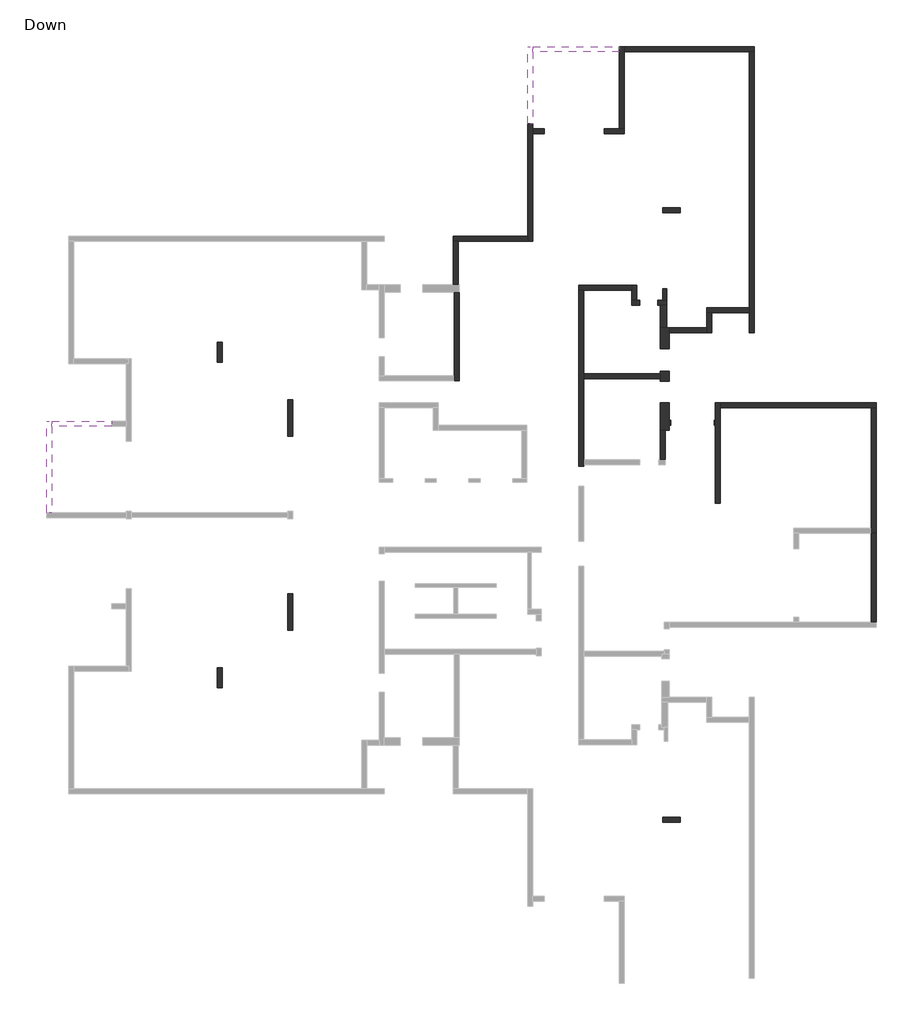
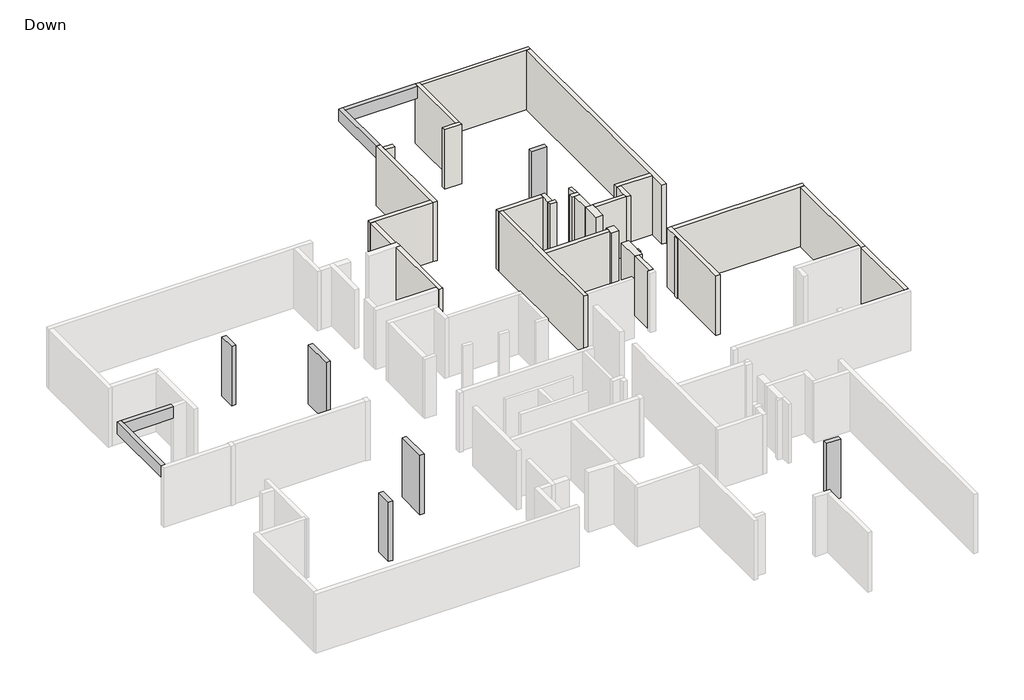
# One storey, part 3 of 3: 30 walls, 6 columns, 4 beams.
"""IFC4 building model written with IfcOpenShell, lengths in millimetres."""

import ifcopenshell
import ifcopenshell.guid

model = None  # the IFC model being written
_history = None  # IfcOwnerHistory: only IFC2X3 demands one
_inside = {}  # id of a spatial element -> (the spatial element, [elements in it])
_under = {}  # id of a project, library or spatial element -> (it, [spatial elements below it])
_declared = {}  # id of a project -> (the project, [libraries it declares])
_typed = {}  # id of a type object -> (the type object, [elements of that type])
_made_of = {}  # id of a material, layer set ... -> (it, [elements and type objects made of it])


def new_model(schema):
    """Start an empty IFC model of exactly this schema.

    Asked for "IFC4X3", IfcOpenShell would pick the latest addendum, in which some entities
    have other attributes; the version numbers below select the first issue.
    IFC2X3 requires an IfcOwnerHistory on every rooted entity: one is made here for all.
    """
    global model, _history
    if schema == "IFC4X3":
        model = ifcopenshell.file(schema_version=(4, 3, 0, 0))
    else:
        model = ifcopenshell.file(schema=schema)
    _inside.clear()
    _under.clear()
    _declared.clear()
    _typed.clear()
    _made_of.clear()
    _history = None
    if model.schema == "IFC2X3":
        org = make("IfcOrganization", Name="unknown")
        user = make(
            "IfcPersonAndOrganization",
            ThePerson=make("IfcPerson", FamilyName="unknown"),
            TheOrganization=org,
        )
        app = make(
            "IfcApplication",
            ApplicationDeveloper=org,
            Version="unknown",
            ApplicationFullName="unknown",
            ApplicationIdentifier="unknown",
        )
        _history = make(
            "IfcOwnerHistory",
            OwningUser=user,
            OwningApplication=app,
            ChangeAction="ADDED",
            CreationDate=0,
        )
    return model


def make(cls, **values):
    """One entity of the class cls with the attributes given. An attribute that is None is left unset."""
    return model.create_entity(
        cls, **{name: value for name, value in values.items() if value is not None}
    )


def rooted(cls, **values):
    """An entity with a GlobalId (a new one), such as an element, a storey or a relation."""
    return make(cls, GlobalId=ifcopenshell.guid.new(), OwnerHistory=_history, **values)


def si_unit(unit_type, name, prefix=None):
    """IfcSIUnit, for example si_unit("LENGTHUNIT", "METRE", prefix="MILLI")."""
    return make("IfcSIUnit", UnitType=unit_type, Prefix=prefix, Name=name)


def assignment(units):
    """IfcUnitAssignment: the units of a project."""
    return None if units is None else make("IfcUnitAssignment", Units=units)


def point(xyz):
    """IfcCartesianPoint."""
    return None if xyz is None else make("IfcCartesianPoint", Coordinates=xyz)


def direction(xyz):
    """IfcDirection."""
    return None if xyz is None else make("IfcDirection", DirectionRatios=xyz)


def frame(location, z_axis=None, x_axis=None):
    """IfcAxis2Placement3D, a coordinate frame: its origin and axes. An axis left out is left unset."""
    return make(
        "IfcAxis2Placement3D",
        Location=point(location),
        Axis=direction(z_axis),
        RefDirection=direction(x_axis),
    )


def origin():
    """The frame at (0, 0, 0) with its axes left unset."""
    return frame((0.0, 0.0, 0.0))


def place(relative_to, where):
    """IfcLocalPlacement: puts the frame where relative to a parent placement (None: the world)."""
    return make(
        "IfcLocalPlacement", PlacementRelTo=relative_to, RelativePlacement=where
    )


def context(
    kind, dimensions, precision=None, world=None, true_north=None, identifier=None
):
    """IfcGeometricRepresentationContext, for example the 3D "Model" context."""
    return make(
        "IfcGeometricRepresentationContext",
        ContextIdentifier=identifier,
        ContextType=kind,
        CoordinateSpaceDimension=dimensions,
        Precision=precision,
        WorldCoordinateSystem=world,
        TrueNorth=true_north,
    )


def project(units=None, contexts=None):
    """IfcProject with its units and contexts."""
    return rooted(
        "IfcProject",
        Name="project",
        RepresentationContexts=contexts,
        UnitsInContext=assignment(units),
    )


def spatial(cls, under=None, at=None, **own):
    """A site, building, storey or space (cls), placed at a placement, below another one or the project."""
    s = rooted(cls, ObjectPlacement=at, **own)
    if under is not None:
        _under.setdefault(under.id(), (under, []))[1].append(s)
    return s


def faces_of(points, faces, orient=None, outer=None):
    """IfcFace entities. A face is a list of loops; a loop is a list of indices into points, from 0.

    orient and outer hold one flag for each loop. By default every Orientation is true, the
    first loop of a face is its IfcFaceOuterBound and the others are IfcFaceBound.
    """
    made = []
    for i, loops in enumerate(faces):
        bounds = []
        for j, loop in enumerate(loops):
            is_outer = j == 0 if outer is None else outer[i][j]
            bounds.append(
                make(
                    "IfcFaceOuterBound" if is_outer else "IfcFaceBound",
                    Bound=make("IfcPolyLoop", Polygon=[points[k] for k in loop]),
                    Orientation=True if orient is None else orient[i][j],
                )
            )
        made.append(make("IfcFace", Bounds=bounds))
    return made


def faceted_brep(points, faces, orient=None, outer=None, voids=None):
    """IfcFacetedBrep: a solid bounded by flat faces; with voids (closed shells), ...WithVoids."""
    shared = [point(p) for p in points]
    hull = make("IfcClosedShell", CfsFaces=faces_of(shared, faces, orient, outer))
    if voids is None:
        return make("IfcFacetedBrep", Outer=hull)
    return make(
        "IfcFacetedBrepWithVoids",
        Outer=hull,
        Voids=[
            make(cls, CfsFaces=faces_of(shared, fs, o, b)) for cls, fs, o, b in voids
        ],
    )


def shape(context_of_items, identifier, shape_type, items):
    """IfcShapeRepresentation: the items that make up one representation, for example the "Body"."""
    return make(
        "IfcShapeRepresentation",
        ContextOfItems=context_of_items,
        RepresentationIdentifier=identifier,
        RepresentationType=shape_type,
        Items=items,
    )


def made_of(thing, what):
    """Note that an element or type object is made of a material, layer set ...; save() writes the relation."""
    if what is not None:
        _made_of.setdefault(what.id(), (what, []))[1].append(thing)
    return thing


def element(
    cls,
    number,
    at=None,
    inside=None,
    cuts=None,
    type_object=None,
    material=None,
    context=None,
    identifier="Body",
    shape_type=None,
    held_by="IfcProductDefinitionShape",
    body=None,
    shapes=None,
    **own,
):
    """One element of the class cls, such as IfcWall. Its Tag is "e" and its number.

    at: its placement. inside: the storey or other place that contains it. cuts: it is an
    opening in that element (IfcRelVoidsElement). A single representation is given by context,
    identifier, shape_type and body (its items); several are given by shapes. held_by: the class
    of the entity that holds the representations. save() writes the other relations.
    """
    e = rooted(cls, Tag="e%d" % number, ObjectPlacement=at, **own)
    if body is not None:
        shapes = [shape(context, identifier, shape_type, body)]
    if shapes is not None:
        e.Representation = make(held_by, Representations=shapes)
    if inside is not None:
        _inside.setdefault(inside.id(), (inside, []))[1].append(e)
    if cuts is not None:
        rooted(
            "IfcRelVoidsElement", RelatingBuildingElement=cuts, RelatedOpeningElement=e
        )
    if type_object is not None:
        _typed.setdefault(type_object.id(), (type_object, []))[1].append(e)
    return made_of(e, material)


def aggregate(whole, parts):
    """IfcRelAggregates: a whole, such as a stair, and the parts it consists of."""
    return rooted("IfcRelAggregates", RelatingObject=whole, RelatedObjects=parts)


def save(model, path):
    """Write the relations noted so far, then the file.

    IfcRelAggregates (storeys below a building ...), IfcRelContainedInSpatialStructure (elements
    in a storey), IfcRelDefinesByType, IfcRelAssociatesMaterial and IfcRelDeclares: one each for
    every whole, place, type object, material and project.
    """
    for whole, parts in _under.values():
        aggregate(whole, parts)
    for where, things in _inside.values():
        rooted(
            "IfcRelContainedInSpatialStructure",
            RelatedElements=things,
            RelatingStructure=where,
        )
    for kind, things in _typed.values():
        rooted("IfcRelDefinesByType", RelatedObjects=things, RelatingType=kind)
    for what, things in _made_of.values():
        rooted("IfcRelAssociatesMaterial", RelatedObjects=things, RelatingMaterial=what)
    for by, libraries in _declared.values():
        rooted("IfcRelDeclares", RelatingContext=by, RelatedDefinitions=libraries)
    model.write(path)


model = new_model("IFC4")

# Units and contexts
model_context = context("Model", 3, world=origin())
ifc_project = project(units=[si_unit("LENGTHUNIT", "METRE", prefix="MILLI")], contexts=[model_context])

# Site, building, storey
site = spatial("IfcSite", under=ifc_project)
building = spatial("IfcBuilding", under=site)
storey = spatial("IfcBuildingStorey", under=building, Name="Down", Elevation=0.0)

# Beams
placement = place(None, origin())
element("IfcBeam", 1, ObjectType="Concrete Rectengular Beam : 20/60", at=placement, inside=storey, context=model_context, shape_type="Brep", body=[
    faceted_brep([(-15742.9172386, 7428.4299293, 3000.0), (-15942.9172386, 7428.4299293, 3000.0), (-15942.9172386, 3770.6507339, 3000.0), (-15742.9172386, 3770.6507339, 3000.0), (-15742.9172386, 7228.4299293, 3000.0), (-15742.9172386, 7428.4299293, 2400.0), (-15742.9172386, 3770.6507339, 2800.0), (-15742.9172386, 3770.6507339, 2400.0), (-15742.9172386, 7228.4299293, 2400.0), (-15942.9172386, 7428.4299293, 2400.0), (-15942.9172386, 3770.6507339, 2400.0)], [[[0, 1, 2, 3, 4]], [[5, 0, 4, 3, 6, 7, 8]], [[9, 5, 8, 7, 10]], [[1, 9, 10, 2]], [[3, 2, 10, 7, 6]], [[1, 0, 5, 9]]]),
])
element("IfcBeam", 2, ObjectType="Concrete Rectengular Beam : 20/60", at=placement, inside=storey, context=model_context, shape_type="Brep", body=[
    faceted_brep([(-15742.9172386, 7428.4299293, 3000.0), (-15742.9172386, 7228.4299293, 3000.0), (-13340.0412254, 7228.4299293, 3000.0), (-13340.0412254, 7428.4299293, 3000.0), (-15742.9172386, 7228.4299293, 2800.0), (-15742.9172386, 7228.4299293, 2400.0), (-13340.0412254, 7228.4299293, 2400.0), (-15742.9172386, 7428.4299293, 2400.0), (-13340.0412254, 7428.4299293, 2400.0)], [[[0, 1, 2, 3]], [[1, 4, 5, 6, 2]], [[5, 7, 8, 6]], [[7, 0, 3, 8]], [[1, 0, 7, 5, 4]], [[3, 2, 6, 8]]]),
])
element("IfcBeam", 3, ObjectType="Concrete Rectengular Beam : 20/60", at=placement, inside=storey, context=model_context, shape_type="Brep", body=[
    faceted_brep([(3525.3580541, 22423.7916826, 3000.0), (3325.3580541, 22423.7916826, 3000.0), (3325.3580541, 19323.9567982, 3000.0), (3525.3580541, 19323.9567982, 3000.0), (3525.3580541, 22223.7916826, 3000.0), (3525.3580541, 22423.7916826, 2400.0), (3525.3580541, 19323.9567982, 2400.0), (3525.3580541, 22223.7916826, 2400.0), (3325.3580541, 22423.7916826, 2400.0), (3325.3580541, 19323.9567982, 2400.0)], [[[0, 1, 2, 3, 4]], [[5, 0, 4, 3, 6, 7]], [[8, 5, 7, 6, 9]], [[1, 8, 9, 2]], [[1, 0, 5, 8]], [[3, 2, 9, 6]]]),
])
element("IfcBeam", 4, ObjectType="Concrete Rectengular Beam : 20/60", at=placement, inside=storey, context=model_context, shape_type="Brep", body=[
    faceted_brep([(6985.0248209, 22223.7916826, 3000.0), (6985.0248209, 22423.7916826, 3000.0), (3525.3580541, 22423.7916826, 3000.0), (3525.3580541, 22223.7916826, 3000.0), (6985.0248209, 22223.7916826, 2400.0), (6985.0248209, 22223.7916826, 2800.0), (3525.3580541, 22223.7916826, 2800.0), (3525.3580541, 22223.7916826, 2400.0), (6985.0248209, 22423.7916826, 2400.0), (3525.3580541, 22423.7916826, 2400.0)], [[[0, 1, 2, 3]], [[4, 5, 0, 3, 6, 7]], [[8, 4, 7, 9]], [[1, 8, 9, 2]], [[1, 0, 5, 4, 8]], [[3, 2, 9, 7, 6]]]),
])

# Columns
element("IfcColumn", 5, ObjectType="Concrete Rectengular Column : 20/147", at=placement, inside=storey, context=model_context, shape_type="Brep", body=[
    faceted_brep([(-6084.7852962, 8293.1687465, 0.0), (-6084.7852962, 6823.1687465, 0.0), (-6284.7852962, 6823.1687465, 0.0), (-6284.7852962, 8293.1687465, 0.0), (-6084.7852962, 8293.1687465, 3000.0), (-6084.7852962, 8090.8811452, 3000.0), (-6084.7852962, 7023.3338621, 3000.0), (-6084.7852962, 6823.1687465, 3000.0), (-6084.7852962, 6823.1687465, 2800.0), (-6084.7852962, 8293.1687465, 2800.0), (-6284.7852962, 6823.1687465, 3000.0), (-6284.7852962, 6823.1687465, 2800.0), (-6284.7852962, 8293.1687465, 3000.0), (-6284.7852962, 8293.1687465, 2800.0)], [[[0, 1, 2, 3]], [[4, 5, 6, 7, 8, 1, 0, 9]], [[7, 10, 11, 2, 1, 8]], [[10, 12, 13, 3, 2, 11]], [[12, 4, 9, 0, 3, 13]], [[4, 12, 10, 7, 6, 5]]]),
])
element("IfcColumn", 6, ObjectType="Concrete Rectengular Column : 20/147", at=placement, inside=storey, context=model_context, shape_type="Brep", body=[
    faceted_brep([(-6084.7852962, -947.1014426, 0.0), (-6284.7852962, -947.1014426, 0.0), (-6284.7852962, 522.8985574, 0.0), (-6084.7852962, 522.8985574, 0.0), (-6084.7852962, -947.1014426, 3000.0), (-6084.7852962, -947.1014426, 2800.0), (-6084.7852962, 522.8985574, 2800.0), (-6084.7852962, 522.8985574, 3000.0), (-6084.7852962, 322.7334418, 3000.0), (-6084.7852962, -744.8138413, 3000.0), (-6284.7852962, 522.8985574, 2800.0), (-6284.7852962, 522.8985574, 3000.0), (-6284.7852962, -947.1014426, 2800.0), (-6284.7852962, -947.1014426, 3000.0)], [[[0, 1, 2, 3]], [[4, 5, 0, 3, 6, 7, 8, 9]], [[7, 6, 3, 2, 10, 11]], [[11, 10, 2, 1, 12, 13]], [[13, 12, 1, 0, 5, 4]], [[4, 9, 8, 7, 11, 13]]]),
])
element("IfcColumn", 7, ObjectType="Concrete Rectengular Column : 20/70", at=placement, inside=storey, context=model_context, shape_type="Brep", body=[
    faceted_brep([(8730.3940793, 15973.4089146, 0.0), (9430.3940793, 15973.4089146, 0.0), (9430.3940793, 15773.4089146, 0.0), (8730.3940793, 15773.4089146, 0.0), (8730.3940793, 15973.4089146, 3000.0), (9430.3940793, 15973.4089146, 3000.0), (9430.3940793, 15973.4089146, 2800.0), (8730.3940793, 15973.4089146, 2800.0), (9430.3940793, 15773.4089146, 3000.0), (9430.3940793, 15773.4089146, 2800.0), (8730.3940793, 15773.4089146, 3000.0), (8730.3940793, 15773.4089146, 2800.0)], [[[0, 1, 2, 3]], [[4, 5, 6, 1, 0, 7]], [[5, 8, 9, 2, 1, 6]], [[8, 10, 11, 3, 2, 9]], [[10, 4, 7, 0, 3, 11]], [[4, 10, 8, 5]]]),
])
element("IfcColumn", 8, ObjectType="Concrete Rectengular Column : 20/70", at=placement, inside=storey, context=model_context, shape_type="Brep", body=[
    faceted_brep([(8730.3940793, -8627.3416107, 0.0), (8730.3940793, -8427.3416107, 0.0), (9430.3940793, -8427.3416107, 0.0), (9430.3940793, -8627.3416107, 0.0), (8730.3940793, -8627.3416107, 3000.0), (8730.3940793, -8627.3416107, 2800.0), (9430.3940793, -8627.3416107, 2800.0), (9430.3940793, -8627.3416107, 3000.0), (9430.3940793, -8427.3416107, 2800.0), (9430.3940793, -8427.3416107, 3000.0), (8730.3940793, -8427.3416107, 2800.0), (8730.3940793, -8427.3416107, 3000.0)], [[[0, 1, 2, 3]], [[4, 5, 0, 3, 6, 7]], [[7, 6, 3, 2, 8, 9]], [[9, 8, 2, 1, 10, 11]], [[11, 10, 1, 0, 5, 4]], [[4, 7, 9, 11]]]),
])
element("IfcColumn", 9, ObjectType="Concrete Rectengular Column : 20/80", at=placement, inside=storey, context=model_context, shape_type="Brep", body=[
    faceted_brep([(-8908.7851697, 10579.8357571, 0.0), (-8908.7851697, 9779.8357571, 0.0), (-9108.7851697, 9779.8357571, 0.0), (-9108.7851697, 10579.8357571, 0.0), (-8908.7851697, 10579.8357571, 3000.0), (-8908.7851697, 9779.8357571, 3000.0), (-8908.7851697, 9779.8357571, 2800.0), (-8908.7851697, 10579.8357571, 2800.0), (-9108.7851697, 9779.8357571, 3000.0), (-9108.7851697, 9779.8357571, 2800.0), (-9108.7851697, 10579.8357571, 3000.0), (-9108.7851697, 10579.8357571, 2800.0)], [[[0, 1, 2, 3]], [[4, 5, 6, 1, 0, 7]], [[5, 8, 9, 2, 1, 6]], [[8, 10, 11, 3, 2, 9]], [[10, 4, 7, 0, 3, 11]], [[4, 10, 8, 5]]]),
])
element("IfcColumn", 10, ObjectType="Concrete Rectengular Column : 20/80", at=placement, inside=storey, context=model_context, shape_type="Brep", body=[
    faceted_brep([(-8908.7851697, -3233.7684532, 0.0), (-9108.7851697, -3233.7684532, 0.0), (-9108.7851697, -2433.7684532, 0.0), (-8908.7851697, -2433.7684532, 0.0), (-8908.7851697, -3233.7684532, 3000.0), (-8908.7851697, -3233.7684532, 2800.0), (-8908.7851697, -2433.7684532, 2800.0), (-8908.7851697, -2433.7684532, 3000.0), (-9108.7851697, -2433.7684532, 2800.0), (-9108.7851697, -2433.7684532, 3000.0), (-9108.7851697, -3233.7684532, 2800.0), (-9108.7851697, -3233.7684532, 3000.0)], [[[0, 1, 2, 3]], [[4, 5, 0, 3, 6, 7]], [[7, 6, 3, 2, 8, 9]], [[9, 8, 2, 1, 10, 11]], [[11, 10, 1, 0, 5, 4]], [[4, 7, 9, 11]]]),
])

# Walls
element("IfcWall", 11, ObjectType="15", at=placement, inside=storey, context=model_context, shape_type="Brep", body=[
    faceted_brep([(8729.6510592, 12723.2738201, 0.0), (8729.6510592, 12275.1201125, 0.0), (8729.6510592, 12275.1201125, 2800.0), (8729.6510592, 12275.1201125, 3000.0), (8729.6510592, 12723.2738201, 3000.0), (8729.6510592, 12723.2738201, 2800.0), (8879.6510592, 12723.2738201, 0.0), (8879.6510592, 12723.2738201, 2800.0), (8879.6510592, 12723.2738201, 3000.0), (8879.6510592, 12275.1201125, 3000.0), (8879.6510592, 12275.1201125, 0.0)], [[[0, 1, 2, 3, 4, 5]], [[6, 7, 8, 9, 10]], [[1, 0, 6, 10]], [[4, 3, 9, 8]], [[0, 5, 4, 8, 7, 6]], [[3, 2, 1, 10, 9]]]),
])
element("IfcWall", 12, ObjectType="20", at=placement, inside=storey, context=model_context, shape_type="Brep", body=[
    faceted_brep([(3525.3580541, 18923.7916826, 0.0), (3983.0434339, 18923.7916826, 0.0), (3983.0434339, 18923.7916826, 2800.0), (3983.0434339, 18923.7916826, 3000.0), (3525.3580541, 18923.7916826, 3000.0), (3525.3580541, 18923.7916826, 2800.0), (3525.3580541, 19123.7916826, 0.0), (3525.3580541, 19123.7916826, 2800.0), (3525.3580541, 19123.7916826, 3000.0), (3983.0434339, 19123.7916826, 3000.0), (3983.0434339, 19123.7916826, 2800.0), (3983.0434339, 19123.7916826, 0.0)], [[[0, 1, 2, 3, 4, 5]], [[6, 7, 8, 9, 10, 11]], [[1, 0, 6, 11]], [[3, 2, 1, 11, 10, 9]], [[4, 3, 9, 8]], [[0, 5, 4, 8, 7, 6]]]),
])
element("IfcWall", 13, ObjectType="20", at=placement, inside=storey, context=model_context, shape_type="Brep", body=[
    faceted_brep([(6385.0248209, 18923.7916826, 0.0), (7185.0248209, 18923.7916826, 0.0), (7185.0248209, 18923.7916826, 2800.0), (7185.0248209, 18923.7916826, 3000.0), (6385.0248209, 18923.7916826, 3000.0), (6385.0248209, 18923.7916826, 2800.0), (6385.0248209, 19123.7916826, 0.0), (6385.0248209, 19123.7916826, 2800.0), (6385.0248209, 19123.7916826, 3000.0), (6985.0248209, 19123.7916826, 3000.0), (7185.0248209, 19123.7916826, 3000.0), (7185.0248209, 19123.7916826, 0.0), (6985.0248209, 19123.7916826, 0.0)], [[[0, 1, 2, 3, 4, 5]], [[6, 7, 8, 9, 10, 11, 12]], [[1, 0, 6, 12, 11]], [[4, 3, 10, 9, 8]], [[0, 5, 4, 8, 7, 6]], [[3, 2, 1, 11, 10]]]),
])
element("IfcWall", 14, ObjectType="20", at=placement, inside=storey, context=model_context, shape_type="Brep", body=[
    faceted_brep([(7185.0248209, 19123.7916826, 0.0), (7185.0248209, 22223.7916826, 0.0), (7185.0248209, 22423.7916826, 0.0), (7185.0248209, 22423.7916826, 3000.0), (7185.0248209, 22223.7916826, 3000.0), (7185.0248209, 19123.7916826, 3000.0), (6985.0248209, 19123.7916826, 0.0), (6985.0248209, 19123.7916826, 2800.0), (6985.0248209, 19123.7916826, 3000.0), (6985.0248209, 22223.7916826, 3000.0), (6985.0248209, 22423.7916826, 3000.0), (6985.0248209, 22423.7916826, 0.0)], [[[0, 1, 2, 3, 4, 5]], [[6, 7, 8, 9, 10, 11]], [[2, 1, 0, 6, 11]], [[5, 4, 3, 10, 9, 8]], [[0, 5, 8, 7, 6]], [[3, 2, 11, 10]]]),
])
element("IfcWall", 15, ObjectType="20", at=placement, inside=storey, context=model_context, shape_type="Brep", body=[
    faceted_brep([(7185.0248209, 22223.7916826, 0.0), (12185.0248209, 22223.7916826, 0.0), (12385.0248209, 22223.7916826, 0.0), (12385.0248209, 22223.7916826, 3000.0), (12185.0248209, 22223.7916826, 3000.0), (7185.0248209, 22223.7916826, 3000.0), (7185.0248209, 22223.7916826, 2800.0), (7185.0248209, 22423.7916826, 0.0), (7185.0248209, 22423.7916826, 3000.0), (12385.0248209, 22423.7916826, 3000.0), (12385.0248209, 22423.7916826, 0.0)], [[[0, 1, 2, 3, 4, 5, 6]], [[7, 8, 9, 10]], [[2, 1, 0, 7, 10]], [[5, 4, 3, 9, 8]], [[0, 6, 5, 8, 7]], [[3, 2, 10, 9]]]),
])
element("IfcWall", 16, ObjectType="20", at=placement, inside=storey, context=model_context, shape_type="Brep", body=[
    faceted_brep([(12185.0248209, 22223.7916826, 0.0), (12185.0248209, 11972.6546366, 0.0), (12185.0248209, 11772.6546366, 0.0), (12185.0248209, 10973.7916826, 0.0), (12185.0248209, 10973.7916826, 3000.0), (12185.0248209, 11772.6546366, 3000.0), (12185.0248209, 11972.6546366, 3000.0), (12185.0248209, 22223.7916826, 3000.0), (12185.0248209, 22223.7916826, 2800.0), (12385.0248209, 22223.7916826, 0.0), (12385.0248209, 22223.7916826, 3000.0), (12385.0248209, 10973.7916826, 3000.0), (12385.0248209, 10973.7916826, 0.0)], [[[0, 1, 2, 3, 4, 5, 6, 7, 8]], [[9, 10, 11, 12]], [[3, 2, 1, 0, 9, 12]], [[4, 3, 12, 11]], [[7, 6, 5, 4, 11, 10]], [[0, 8, 7, 10, 9]]]),
])
element("IfcWall", 17, ObjectType="20", at=placement, inside=storey, context=model_context, shape_type="Brep", body=[
    faceted_brep([(10478.8780181, 11772.6546366, 0.0), (10678.8780181, 11772.6546366, 0.0), (12185.0248209, 11772.6546366, 0.0), (12185.0248209, 11772.6546366, 3000.0), (10678.8780181, 11772.6546366, 3000.0), (10478.8780181, 11772.6546366, 3000.0), (10478.8780181, 11972.6546366, 0.0), (10478.8780181, 11972.6546366, 2800.0), (10478.8780181, 11972.6546366, 3000.0), (12185.0248209, 11972.6546366, 3000.0), (12185.0248209, 11972.6546366, 2800.0), (12185.0248209, 11972.6546366, 0.0)], [[[0, 1, 2, 3, 4, 5]], [[6, 7, 8, 9, 10, 11]], [[2, 1, 0, 6, 11]], [[5, 4, 3, 9, 8]], [[3, 2, 11, 10, 9]], [[0, 5, 8, 7, 6]]]),
])
element("IfcWall", 18, ObjectType="20", at=placement, inside=storey, context=model_context, shape_type="Brep", body=[
    faceted_brep([(10478.8780181, 11772.6546366, 0.0), (10478.8780181, 11171.8290587, 0.0), (10478.8780181, 10971.8290587, 0.0), (10478.8780181, 10971.8290587, 3000.0), (10478.8780181, 11171.8290587, 3000.0), (10478.8780181, 11772.6546366, 3000.0), (10678.8780181, 11772.6546366, 0.0), (10678.8780181, 11772.6546366, 3000.0), (10678.8780181, 10971.8290587, 3000.0), (10678.8780181, 10971.8290587, 0.0)], [[[0, 1, 2, 3, 4, 5]], [[6, 7, 8, 9]], [[2, 1, 0, 6, 9]], [[5, 4, 3, 8, 7]], [[3, 2, 9, 8]], [[0, 5, 7, 6]]]),
])
element("IfcWall", 19, ObjectType="20", at=placement, inside=storey, context=model_context, shape_type="Brep", body=[
    faceted_brep([(10478.8780181, 11171.8290587, 0.0), (8979.733617, 11171.8290587, 0.0), (8979.733617, 11171.8290587, 3000.0), (10478.8780181, 11171.8290587, 3000.0), (10478.8780181, 11171.8290587, 2800.0), (10478.8780181, 10971.8290587, 0.0), (10478.8780181, 10971.8290587, 3000.0), (8979.733617, 10971.8290587, 3000.0), (8979.733617, 10971.8290587, 0.0)], [[[0, 1, 2, 3, 4]], [[5, 6, 7, 8]], [[1, 0, 5, 8]], [[3, 2, 7, 6]], [[0, 4, 3, 6, 5]], [[2, 1, 8, 7]]]),
])
element("IfcWall", 20, ObjectType="20", at=placement, inside=storey, context=model_context, shape_type="Brep", body=[
    faceted_brep([(7795.7123021, 12275.2852281, 0.0), (7681.1671205, 12275.2852281, 0.0), (7481.1671205, 12275.2852281, 0.0), (7481.1671205, 12275.2852281, 3000.0), (7681.1671205, 12275.2852281, 3000.0), (7795.7123021, 12275.2852281, 3000.0), (7795.7123021, 12275.2852281, 2800.0), (7795.7123021, 12075.2852281, 0.0), (7795.7123021, 12075.2852281, 2800.0), (7795.7123021, 12075.2852281, 3000.0), (7481.1671205, 12075.2852281, 3000.0), (7481.1671205, 12075.2852281, 2800.0), (7481.1671205, 12075.2852281, 0.0), (7795.7123021, 12270.1201125, 3000.0)], [[[0, 1, 2, 3, 4, 5, 6]], [[7, 8, 9, 10, 11, 12]], [[2, 1, 0, 7, 12]], [[5, 4, 3, 10, 9, 13]], [[0, 6, 5, 13, 9, 8, 7]], [[3, 2, 12, 11, 10]]]),
])
element("IfcWall", 21, ObjectType="20", at=placement, inside=storey, context=model_context, shape_type="Brep", body=[
    faceted_brep([(7681.1671205, 12275.2852281, 0.0), (7681.1671205, 12875.7805748, 0.0), (7681.1671205, 12875.7805748, 2800.0), (7681.1671205, 12875.7805748, 3000.0), (7681.1671205, 12275.2852281, 3000.0), (7681.1671205, 12275.2852281, 2800.0), (7481.1671205, 12275.2852281, 0.0), (7481.1671205, 12275.2852281, 3000.0), (7481.1671205, 12675.7805748, 3000.0), (7481.1671205, 12875.7805748, 3000.0), (7481.1671205, 12875.7805748, 0.0), (7481.1671205, 12675.7805748, 0.0)], [[[0, 1, 2, 3, 4, 5]], [[6, 7, 8, 9, 10, 11]], [[1, 0, 6, 11, 10]], [[4, 3, 9, 8, 7]], [[0, 5, 4, 7, 6]], [[3, 2, 1, 10, 9]]]),
])
element("IfcWall", 22, ObjectType="20", at=placement, inside=storey, context=model_context, shape_type="Brep", body=[
    faceted_brep([(7481.1671205, 12875.7805748, 0.0), (5355.6042265, 12875.7805748, 0.0), (5355.6042265, 12875.7805748, 2800.0), (5355.6042265, 12875.7805748, 3000.0), (7481.1671205, 12875.7805748, 3000.0), (7481.1671205, 12675.7805748, 0.0), (7481.1671205, 12675.7805748, 2800.0), (7481.1671205, 12675.7805748, 3000.0), (5555.6042265, 12675.7805748, 3000.0), (5355.6042265, 12675.7805748, 3000.0), (5355.6042265, 12675.7805748, 0.0), (5555.6042265, 12675.7805748, 0.0)], [[[0, 1, 2, 3, 4]], [[5, 6, 7, 8, 9, 10, 11]], [[1, 0, 5, 11, 10]], [[4, 3, 9, 8, 7]], [[0, 4, 7, 6, 5]], [[3, 2, 1, 10, 9]]]),
])
element("IfcWall", 23, ObjectType="20", at=placement, inside=storey, context=model_context, shape_type="Brep", body=[
    faceted_brep([(5355.6042265, 12675.7805748, 0.0), (5355.6042265, 5624.5609711, 0.0), (5355.6042265, 5624.5609711, 2800.0), (5355.6042265, 5624.5609711, 3000.0), (5355.6042265, 9203.7038711, 3000.0), (5355.6042265, 12675.7805748, 3000.0), (5555.6042265, 12675.7805748, 0.0), (5555.6042265, 12675.7805748, 2800.0), (5555.6042265, 12675.7805748, 3000.0), (5555.6042265, 9325.0675757, 3000.0), (5555.6042265, 9125.0675757, 3000.0), (5555.6042265, 5874.60225, 3000.0), (5555.6042265, 5674.60225, 3000.0), (5555.6042265, 5624.5609711, 3000.0), (5555.6042265, 5624.5609711, 2800.0), (5555.6042265, 5624.5609711, 0.0), (5555.6042265, 5674.60225, 0.0), (5555.6042265, 5874.60225, 0.0), (5555.6042265, 9125.0675757, 0.0), (5555.6042265, 9325.0675757, 0.0)], [[[0, 1, 2, 3, 4, 5]], [[6, 7, 8, 9, 10, 11, 12, 13, 14, 15, 16, 17, 18, 19]], [[1, 0, 6, 19, 18, 17, 16, 15]], [[3, 2, 1, 15, 14, 13]], [[5, 4, 3, 13, 12, 11, 10, 9, 8]], [[0, 5, 8, 7, 6]]]),
])
element("IfcWall", 24, ObjectType="20", at=placement, inside=storey, context=model_context, shape_type="Brep", body=[
    faceted_brep([(8829.8987326, 5874.60225, 0.0), (8829.8987326, 7073.375141, 0.0), (8829.8987326, 7073.375141, 2800.0), (8829.8987326, 7073.375141, 3000.0), (8829.8987326, 5874.60225, 3000.0), (8629.8987326, 5874.60225, 0.0), (8629.8987326, 5874.60225, 2800.0), (8629.8987326, 5874.60225, 3000.0), (8629.8987326, 7073.375141, 3000.0), (8629.8987326, 7073.375141, 2800.0), (8629.8987326, 7073.375141, 0.0)], [[[0, 1, 2, 3, 4]], [[5, 6, 7, 8, 9, 10]], [[1, 0, 5, 10]], [[3, 2, 1, 10, 9, 8]], [[4, 3, 8, 7]], [[0, 4, 7, 6, 5]]]),
])
element("IfcWall", 25, ObjectType="20", at=placement, inside=storey, context=model_context, shape_type="Brep", body=[
    faceted_brep([(5555.6042265, 9125.0675757, 0.0), (8629.733617, 9125.0675757, 0.0), (8629.733617, 9125.0675757, 2800.0), (8629.733617, 9125.0675757, 3000.0), (5555.6042265, 9125.0675757, 3000.0), (5555.6042265, 9125.0675757, 2800.0), (5555.6042265, 9325.0675757, 0.0), (5555.6042265, 9325.0675757, 2800.0), (5555.6042265, 9325.0675757, 3000.0), (8629.733617, 9325.0675757, 3000.0), (8629.733617, 9325.0675757, 2800.0), (8629.733617, 9325.0675757, 0.0)], [[[0, 1, 2, 3, 4, 5]], [[6, 7, 8, 9, 10, 11]], [[1, 0, 6, 11]], [[4, 3, 9, 8]], [[0, 5, 4, 8, 7, 6]], [[3, 2, 1, 11, 10, 9]]]),
])
element("IfcWall", 26, ObjectType="20", at=placement, inside=storey, context=model_context, shape_type="Brep", body=[
    faceted_brep([(8979.733617, 7273.7053722, 0.0), (9040.0225693, 7273.7053722, 0.0), (9040.0225693, 7273.7053722, 2800.0), (9040.0225693, 7273.7053722, 3000.0), (8979.733617, 7273.7053722, 3000.0), (8979.733617, 7273.7053722, 2800.0), (8979.733617, 7473.7053722, 0.0), (8979.733617, 7473.7053722, 3000.0), (9040.0225693, 7473.7053722, 3000.0), (9040.0225693, 7473.7053722, 2800.0), (9040.0225693, 7473.7053722, 0.0)], [[[0, 1, 2, 3, 4, 5]], [[6, 7, 8, 9, 10]], [[1, 0, 6, 10]], [[3, 2, 1, 10, 9, 8]], [[4, 3, 8, 7]], [[0, 5, 4, 7, 6]]]),
])
element("IfcWall", 27, ObjectType="20", at=placement, inside=storey, context=model_context, shape_type="Brep", body=[
    faceted_brep([(10774.0296242, 7273.7053722, 0.0), (10824.7313654, 7273.7053722, 0.0), (10824.7313654, 7273.7053722, 2800.0), (10824.7313654, 7273.7053722, 3000.0), (10774.0296242, 7273.7053722, 3000.0), (10774.0296242, 7273.7053722, 2800.0), (10774.0296242, 7473.7053722, 0.0), (10774.0296242, 7473.7053722, 2800.0), (10774.0296242, 7473.7053722, 3000.0), (10824.7313654, 7473.7053722, 3000.0), (10824.7313654, 7473.7053722, 0.0)], [[[0, 1, 2, 3, 4, 5]], [[6, 7, 8, 9, 10]], [[1, 0, 6, 10]], [[4, 3, 9, 8]], [[0, 5, 4, 8, 7, 6]], [[3, 2, 1, 10, 9]]]),
])
element("IfcWall", 28, ObjectType="20", at=placement, inside=storey, context=model_context, shape_type="Brep", body=[
    faceted_brep([(11024.7313654, 4144.7688666, 0.0), (11024.7313654, 7974.2832767, 0.0), (11024.7313654, 8174.2832767, 0.0), (11024.7313654, 8174.2832767, 3000.0), (11024.7313654, 7974.2832767, 3000.0), (11024.7313654, 4144.7688666, 3000.0), (11024.7313654, 4144.7688666, 2800.0), (10824.7313654, 4144.7688666, 0.0), (10824.7313654, 4144.7688666, 2800.0), (10824.7313654, 4144.7688666, 3000.0), (10824.7313654, 7273.7053722, 3000.0), (10824.7313654, 7473.7053722, 3000.0), (10824.7313654, 8174.2832767, 3000.0), (10824.7313654, 8174.2832767, 0.0), (10824.7313654, 7473.7053722, 0.0), (10824.7313654, 7273.7053722, 0.0)], [[[0, 1, 2, 3, 4, 5, 6]], [[7, 8, 9, 10, 11, 12, 13, 14, 15]], [[2, 1, 0, 7, 15, 14, 13]], [[5, 4, 3, 12, 11, 10, 9]], [[0, 6, 5, 9, 8, 7]], [[3, 2, 13, 12]]]),
])
element("IfcWall", 29, ObjectType="20", at=placement, inside=storey, context=model_context, shape_type="Brep", body=[
    faceted_brep([(11024.7313654, 7974.2832767, 0.0), (17074.9602757, 7974.2832767, 0.0), (17274.9602757, 7974.2832767, 0.0), (17274.9602757, 7974.2832767, 3000.0), (17074.9602757, 7974.2832767, 3000.0), (11024.7313654, 7974.2832767, 3000.0), (11024.7313654, 7974.2832767, 2800.0), (11024.7313654, 8174.2832767, 0.0), (11024.7313654, 8174.2832767, 3000.0), (17274.9602757, 8174.2832767, 3000.0), (17274.9602757, 8174.2832767, 0.0)], [[[0, 1, 2, 3, 4, 5, 6]], [[7, 8, 9, 10]], [[2, 1, 0, 7, 10]], [[5, 4, 3, 9, 8]], [[0, 6, 5, 8, 7]], [[3, 2, 10, 9]]]),
])
element("IfcWall", 30, ObjectType="20", at=placement, inside=storey, context=model_context, shape_type="Brep", body=[
    faceted_brep([(17074.9602757, 7974.2832767, 0.0), (17074.9602757, 3143.7781731, 0.0), (17074.9602757, 2943.7781731, 0.0), (17074.9602757, 2943.7781731, 3000.0), (17074.9602757, 3143.7781731, 3000.0), (17074.9602757, 7974.2832767, 3000.0), (17074.9602757, 7974.2832767, 2800.0), (17274.9602757, 7974.2832767, 0.0), (17274.9602757, 7974.2832767, 3000.0), (17274.9602757, 2943.7781731, 3000.0), (17274.9602757, 2943.7781731, 0.0)], [[[0, 1, 2, 3, 4, 5, 6]], [[7, 8, 9, 10]], [[2, 1, 0, 7, 10]], [[5, 4, 3, 9, 8]], [[0, 6, 5, 8, 7]], [[3, 2, 10, 9]]]),
])
element("IfcWall", 31, ObjectType="20", at=placement, inside=storey, context=model_context, shape_type="Brep", body=[
    faceted_brep([(3325.3580541, 19323.9567982, 0.0), (3325.3580541, 14822.6246156, 0.0), (3325.3580541, 14622.6246156, 0.0), (3325.3580541, 14622.6246156, 3000.0), (3325.3580541, 14822.6246156, 3000.0), (3325.3580541, 19323.9567982, 3000.0), (3325.3580541, 19323.9567982, 2400.0), (3525.3580541, 19323.9567982, 0.0), (3525.3580541, 19323.9567982, 2400.0), (3525.3580541, 19323.9567982, 3000.0), (3525.3580541, 19123.7916826, 3000.0), (3525.3580541, 18923.7916826, 3000.0), (3525.3580541, 14622.6246156, 3000.0), (3525.3580541, 14622.6246156, 2800.0), (3525.3580541, 14622.6246156, 0.0), (3525.3580541, 18923.7916826, 0.0), (3525.3580541, 19123.7916826, 0.0)], [[[0, 1, 2, 3, 4, 5, 6]], [[7, 8, 9, 10, 11, 12, 13, 14, 15, 16]], [[2, 1, 0, 7, 16, 15, 14]], [[5, 4, 3, 12, 11, 10, 9]], [[0, 6, 5, 9, 8, 7]], [[3, 2, 14, 13, 12]]]),
])
element("IfcWall", 32, ObjectType="20", at=placement, inside=storey, context=model_context, shape_type="Brep", body=[
    faceted_brep([(3325.3580541, 14822.6246156, 0.0), (339.5617467, 14822.6246156, 0.0), (339.5617467, 14822.6246156, 3000.0), (3325.3580541, 14822.6246156, 3000.0), (3325.3580541, 14622.6246156, 0.0), (3325.3580541, 14622.6246156, 3000.0), (539.5617467, 14622.6246156, 3000.0), (339.5617467, 14622.6246156, 3000.0), (339.5617467, 14622.6246156, 0.0), (539.5617467, 14622.6246156, 0.0)], [[[0, 1, 2, 3]], [[4, 5, 6, 7, 8, 9]], [[1, 0, 4, 9, 8]], [[3, 2, 7, 6, 5]], [[2, 1, 8, 7]], [[0, 3, 5, 4]]]),
])
element("IfcWall", 33, ObjectType="20", at=placement, inside=storey, context=model_context, shape_type="Brep", body=[
    faceted_brep([(339.5617467, 14622.6246156, 0.0), (339.5617467, 12892.2958855, 0.0), (339.5617467, 12892.2958855, 3000.0), (339.5617467, 14622.6246156, 3000.0), (539.5617467, 14622.6246156, 0.0), (539.5617467, 14622.6246156, 2800.0), (539.5617467, 14622.6246156, 3000.0), (539.5617467, 12892.2958855, 3000.0), (539.5617467, 12892.2958855, 2800.0), (539.5617467, 12892.2958855, 0.0)], [[[0, 1, 2, 3]], [[4, 5, 6, 7, 8, 9]], [[1, 0, 4, 9]], [[3, 2, 7, 6]], [[0, 3, 6, 5, 4]], [[2, 1, 9, 8, 7]]]),
])
element("IfcWall", 34, ObjectType="20", at=placement, inside=storey, context=model_context, shape_type="Brep", body=[
    faceted_brep([(385.0023051, 12592.2958855, 0.0), (385.0023051, 9253.5800344, 0.0), (385.0023051, 9053.5800344, 0.0), (385.0023051, 9053.5800344, 3000.0), (385.0023051, 9253.5800344, 3000.0), (385.0023051, 12592.2958855, 3000.0), (385.0023051, 12592.2958855, 2800.0), (585.0023051, 12592.2958855, 0.0), (585.0023051, 12592.2958855, 3000.0), (585.0023051, 9203.7038711, 3000.0), (585.0023051, 9053.5800344, 3000.0), (585.0023051, 9053.5800344, 2800.0), (585.0023051, 9053.5800344, 0.0)], [[[0, 1, 2, 3, 4, 5, 6]], [[7, 8, 9, 10, 11, 12]], [[2, 1, 0, 7, 12]], [[5, 4, 3, 10, 9, 8]], [[0, 6, 5, 8, 7]], [[3, 2, 12, 11, 10]]]),
])
element("IfcWall", 35, ObjectType="20", at=placement, inside=storey, context=model_context, shape_type="Brep", body=[
    faceted_brep([(17274.9602757, -628.2159728, 0.0), (17274.9602757, 2943.7781731, 0.0), (17274.9602757, 2943.7781731, 3000.0), (17274.9602757, -628.2159728, 3000.0), (17074.9602757, -628.2159728, 0.0), (17074.9602757, -628.2159728, 2800.0), (17074.9602757, -628.2159728, 3000.0), (17074.9602757, 2943.7781731, 3000.0), (17074.9602757, 2943.7781731, 2800.0), (17074.9602757, 2943.7781731, 0.0)], [[[0, 1, 2, 3]], [[4, 5, 6, 7, 8, 9]], [[1, 0, 4, 9]], [[3, 2, 7, 6]], [[0, 3, 6, 5, 4]], [[2, 1, 9, 8, 7]]]),
])
element("IfcWall", 36, ObjectType="20", at=placement, inside=storey, context=model_context, shape_type="Brep", body=[
    faceted_brep([(8530.0225693, 12075.1201125, 0.0), (8629.733617, 12075.1201125, 0.0), (8879.6510592, 12075.1201125, 0.0), (8879.6510592, 12075.1201125, 3000.0), (8629.733617, 12075.1201125, 3000.0), (8530.0225693, 12075.1201125, 3000.0), (8530.0225693, 12075.1201125, 2800.0), (8530.0225693, 12275.1201125, 0.0), (8530.0225693, 12275.1201125, 2800.0), (8530.0225693, 12275.1201125, 3000.0), (8729.6510592, 12275.1201125, 3000.0), (8879.6510592, 12275.1201125, 3000.0), (8879.6510592, 12275.1201125, 0.0), (8729.6510592, 12275.1201125, 0.0), (8530.0225693, 12270.1201125, 3000.0)], [[[0, 1, 2, 3, 4, 5, 6]], [[7, 8, 9, 10, 11, 12, 13]], [[2, 1, 0, 7, 13, 12]], [[5, 4, 3, 11, 10, 9, 14]], [[0, 6, 5, 14, 9, 8, 7]], [[3, 2, 12, 11]]]),
])
element("IfcWall", 37, ObjectType="25", at=placement, inside=storey, context=model_context, shape_type="Brep", body=[
    faceted_brep([(8879.733617, 11171.8290587, 0.0), (8879.733617, 12075.1201125, 0.0), (8879.733617, 12075.1201125, 3000.0), (8879.733617, 11171.8290587, 3000.0), (8879.733617, 11171.8290587, 2800.0), (8629.733617, 11171.8290587, 0.0), (8629.733617, 11171.8290587, 3000.0), (8629.733617, 12075.1201125, 3000.0), (8629.733617, 12075.1201125, 2800.0), (8629.733617, 12075.1201125, 0.0)], [[[0, 1, 2, 3, 4]], [[5, 6, 7, 8, 9]], [[1, 0, 5, 9]], [[3, 2, 7, 6]], [[0, 4, 3, 6, 5]], [[2, 1, 9, 8, 7]]]),
])
element("IfcWall", 38, ObjectType="35", at=placement, inside=storey, context=model_context, shape_type="Brep", body=[
    faceted_brep([(8979.733617, 10323.6753511, 0.0), (8979.733617, 10971.8290587, 0.0), (8979.733617, 11171.8290587, 0.0), (8979.733617, 11171.8290587, 3000.0), (8979.733617, 10971.8290587, 3000.0), (8979.733617, 10323.6753511, 3000.0), (8979.733617, 10323.6753511, 2800.0), (8629.733617, 10323.6753511, 0.0), (8629.733617, 10323.6753511, 2800.0), (8629.733617, 10323.6753511, 3000.0), (8629.733617, 11171.8290587, 3000.0), (8629.733617, 11171.8290587, 0.0), (8879.733617, 11171.8290587, 0.0), (8879.733617, 11171.8290587, 3000.0)], [[[0, 1, 2, 3, 4, 5, 6]], [[7, 8, 9, 10, 11]], [[2, 1, 0, 7, 11, 12]], [[5, 4, 3, 13, 10, 9]], [[0, 6, 5, 9, 8, 7]], [[3, 2, 12, 11, 10, 13]]]),
])
element("IfcWall", 39, ObjectType="35", at=placement, inside=storey, context=model_context, shape_type="Brep", body=[
    faceted_brep([(8979.733617, 9024.9850179, 0.0), (8979.733617, 9425.3152491, 0.0), (8979.733617, 9425.3152491, 2800.0), (8979.733617, 9425.3152491, 3000.0), (8979.733617, 9024.9850179, 3000.0), (8979.733617, 9024.9850179, 2800.0), (8629.733617, 9024.9850179, 0.0), (8629.733617, 9024.9850179, 2800.0), (8629.733617, 9024.9850179, 3000.0), (8629.733617, 9125.0675757, 3000.0), (8629.733617, 9325.0675757, 3000.0), (8629.733617, 9425.3152491, 3000.0), (8629.733617, 9425.3152491, 2800.0), (8629.733617, 9425.3152491, 0.0), (8629.733617, 9325.0675757, 0.0), (8629.733617, 9125.0675757, 0.0)], [[[0, 1, 2, 3, 4, 5]], [[6, 7, 8, 9, 10, 11, 12, 13, 14, 15]], [[1, 0, 6, 15, 14, 13]], [[3, 2, 1, 13, 12, 11]], [[4, 3, 11, 10, 9, 8]], [[0, 5, 4, 8, 7, 6]]]),
])
element("IfcWall", 40, ObjectType="35", at=placement, inside=storey, context=model_context, shape_type="Brep", body=[
    faceted_brep([(8629.733617, 8174.2832767, 0.0), (8629.733617, 7073.375141, 0.0), (8629.733617, 7073.375141, 2800.0), (8629.733617, 7073.375141, 3000.0), (8629.733617, 8174.2832767, 3000.0), (8629.733617, 8174.2832767, 2800.0), (8979.733617, 8174.2832767, 0.0), (8979.733617, 8174.2832767, 2800.0), (8979.733617, 8174.2832767, 3000.0), (8979.733617, 7473.7053722, 3000.0), (8979.733617, 7273.7053722, 3000.0), (8979.733617, 7073.375141, 3000.0), (8979.733617, 7073.375141, 2800.0), (8979.733617, 7073.375141, 0.0), (8979.733617, 7273.7053722, 0.0), (8979.733617, 7473.7053722, 0.0), (8829.8987326, 7073.375141, 0.0), (8629.8987326, 7073.375141, 0.0), (8829.8987326, 7073.375141, 3000.0), (8629.8987326, 7073.375141, 3000.0)], [[[0, 1, 2, 3, 4, 5]], [[6, 7, 8, 9, 10, 11, 12, 13, 14, 15]], [[1, 0, 6, 15, 14, 13, 16, 17]], [[3, 2, 1, 17, 16, 13, 12, 11, 18, 19]], [[4, 3, 19, 18, 11, 10, 9, 8]], [[0, 5, 4, 8, 7, 6]]]),
])

save(model, "model.ifc")

# Revit data of these elements
# Type "Concrete Rectengular Beam : 20/60"
#   Length [instance default] = 152.4 cm
#   b = 20 cm
#   h = 60 cm
#   Structural Material [instance default] = Concrete
#   Assembly Code = ""
# Type "Concrete Rectengular Column : 20/147"
#   b = 20 cm
#   h = 147 cm
#   Structural Material [instance default] = Concrete
# Type "Concrete Rectengular Column : 20/70"
#   b = 20 cm
#   h = 70 cm
#   Structural Material [instance default] = Concrete
# Type "Concrete Rectengular Column : 20/80"
#   b = 20 cm
#   h = 80 cm
#   Structural Material [instance default] = Concrete
# Type "15"
#   Layers, outside or top first: 15 cm "Concrete" (function 1)
# Type "20"
#   Layers, outside or top first: 20 cm "Concrete" (function 1)
# Type "25"
#   Layers, outside or top first: 25 cm "Concrete" (function 1)
# Type "35"
#   Layers, outside or top first: 35 cm "Concrete" (function 1)
# Element 1 (IfcBeam, "Concrete Rectengular Beam : 20/60")
#   Comments = ""
#   Mark = "B1"
#   SOFiSTiK_AMG_Comments = ""
#   SOFiSTiK_AMG_Scheduled = yes
#   SOFiSTiK_AMG_Adjusted = yes
#   Structural Material = Concrete
#   Phase Created = New Construction
#   Materials on its faces: "Concrete"
# Element 2 (IfcBeam, "Concrete Rectengular Beam : 20/60")
#   Comments = ""
#   Mark = "B2"
#   SOFiSTiK_AMG_Comments = ""
#   SOFiSTiK_AMG_Scheduled = yes
#   SOFiSTiK_AMG_Adjusted = yes
#   Structural Material = Concrete
#   Phase Created = New Construction
#   Materials on its faces: "Concrete"
# Element 3 (IfcBeam, "Concrete Rectengular Beam : 20/60")
#   Comments = ""
#   Mark = "B3"
#   SOFiSTiK_AMG_Comments = ""
#   SOFiSTiK_AMG_Scheduled = yes
#   SOFiSTiK_AMG_Adjusted = yes
#   Structural Material = Concrete
#   Phase Created = New Construction
#   Materials on its faces: "Concrete"
# Element 4 (IfcBeam, "Concrete Rectengular Beam : 20/60")
#   Comments = ""
#   Mark = "B4"
#   SOFiSTiK_AMG_Comments = ""
#   SOFiSTiK_AMG_Scheduled = yes
#   SOFiSTiK_AMG_Adjusted = yes
#   Structural Material = Concrete
#   Phase Created = New Construction
#   Materials on its faces: "Concrete"
# Element 5 (IfcColumn, "Concrete Rectengular Column : 20/147")
#   Comments = ""
#   Mark = "C1"
#   SOFiSTiK_AMG_Comments = ""
#   SOFiSTiK_AMG_Scheduled = yes
#   SOFiSTiK_AMG_Adjusted = yes
#   Structural Material = Concrete
#   Phase Created = New Construction
#   Materials on its faces: "Concrete"
# Element 6 (IfcColumn, "Concrete Rectengular Column : 20/147")
#   Comments = ""
#   Mark = "C2"
#   SOFiSTiK_AMG_Comments = ""
#   SOFiSTiK_AMG_Scheduled = yes
#   SOFiSTiK_AMG_Adjusted = yes
#   Structural Material = Concrete
#   Phase Created = New Construction
#   Materials on its faces: "Concrete"
# Element 7 (IfcColumn, "Concrete Rectengular Column : 20/70")
#   Comments = ""
#   Mark = "C3"
#   SOFiSTiK_AMG_Comments = ""
#   SOFiSTiK_AMG_Scheduled = yes
#   SOFiSTiK_AMG_Adjusted = yes
#   Structural Material = Concrete
#   Phase Created = New Construction
#   Materials on its faces: "Concrete"
# Element 8 (IfcColumn, "Concrete Rectengular Column : 20/70")
#   Comments = ""
#   Mark = "C4"
#   SOFiSTiK_AMG_Comments = ""
#   SOFiSTiK_AMG_Scheduled = yes
#   SOFiSTiK_AMG_Adjusted = yes
#   Structural Material = Concrete
#   Phase Created = New Construction
#   Materials on its faces: "Concrete"
# Element 9 (IfcColumn, "Concrete Rectengular Column : 20/80")
#   Comments = ""
#   Mark = "C5"
#   SOFiSTiK_AMG_Comments = ""
#   SOFiSTiK_AMG_Scheduled = yes
#   SOFiSTiK_AMG_Adjusted = yes
#   Structural Material = Concrete
#   Phase Created = New Construction
#   Materials on its faces: "Concrete"
# Element 10 (IfcColumn, "Concrete Rectengular Column : 20/80")
#   Comments = ""
#   Mark = "C6"
#   SOFiSTiK_AMG_Comments = ""
#   SOFiSTiK_AMG_Scheduled = yes
#   SOFiSTiK_AMG_Adjusted = yes
#   Structural Material = Concrete
#   Phase Created = New Construction
#   Materials on its faces: "Concrete"
# Element 11 (IfcWall, "15")
#   Comments = ""
#   Mark = "W99"
#   SOFiSTiK_EdgeZones = "W99"
#   SOFiSTiK_AMG_Comments = ""
#   Top Offset = 0 cm
#   Base Offset = 0 cm
#   wall height = 300 cm
#   SOFiSTiK_AMG_Scheduled = yes
#   SOFiSTiK_AMG_Adjusted = yes
#   Phase Created = New Construction
#   Base Constraint = Down
#   Top Constraint = Typical Floor
#   Materials on its faces: "Concrete"
# Element 12 (IfcWall, "20")
#   Comments = ""
#   Mark = "W1"
#   SOFiSTiK_EdgeZones = "W1"
#   SOFiSTiK_AMG_Comments = ""
#   Top Offset = 0 cm
#   Base Offset = 0 cm
#   wall height = 300 cm
#   SOFiSTiK_AMG_Scheduled = yes
#   SOFiSTiK_AMG_Adjusted = yes
#   Phase Created = New Construction
#   Base Constraint = Down
#   Top Constraint = Typical Floor
#   Materials on its faces: "Concrete"
# Element 13 (IfcWall, "20")
#   Comments = ""
#   Mark = "W2"
#   SOFiSTiK_EdgeZones = "W2"
#   SOFiSTiK_AMG_Comments = ""
#   Top Offset = 0 cm
#   Base Offset = 0 cm
#   wall height = 300 cm
#   SOFiSTiK_AMG_Scheduled = yes
#   SOFiSTiK_AMG_Adjusted = yes
#   Phase Created = New Construction
#   Base Constraint = Down
#   Top Constraint = Typical Floor
#   Materials on its faces: "Concrete"
# Element 14 (IfcWall, "20")
#   Comments = ""
#   Mark = "W3"
#   SOFiSTiK_EdgeZones = "W3"
#   SOFiSTiK_AMG_Comments = ""
#   Top Offset = 0 cm
#   Base Offset = 0 cm
#   wall height = 300 cm
#   SOFiSTiK_AMG_Scheduled = yes
#   SOFiSTiK_AMG_Adjusted = yes
#   Phase Created = New Construction
#   Base Constraint = Down
#   Top Constraint = Typical Floor
#   Materials on its faces: "Concrete"
# Element 15 (IfcWall, "20")
#   Comments = ""
#   Mark = "W4"
#   SOFiSTiK_EdgeZones = "W4"
#   SOFiSTiK_AMG_Comments = ""
#   Top Offset = 0 cm
#   Base Offset = 0 cm
#   wall height = 300 cm
#   SOFiSTiK_AMG_Scheduled = yes
#   SOFiSTiK_AMG_Adjusted = yes
#   Phase Created = New Construction
#   Base Constraint = Down
#   Top Constraint = Typical Floor
#   Materials on its faces: "Concrete"
# Element 16 (IfcWall, "20")
#   Comments = ""
#   Mark = "W5"
#   SOFiSTiK_EdgeZones = "W5"
#   SOFiSTiK_AMG_Comments = ""
#   Top Offset = 0 cm
#   Base Offset = 0 cm
#   wall height = 300 cm
#   SOFiSTiK_AMG_Scheduled = yes
#   SOFiSTiK_AMG_Adjusted = yes
#   Phase Created = New Construction
#   Base Constraint = Down
#   Top Constraint = Typical Floor
#   Materials on its faces: "Concrete"
# Element 17 (IfcWall, "20")
#   Comments = ""
#   Mark = "W6"
#   SOFiSTiK_EdgeZones = "W6"
#   SOFiSTiK_AMG_Comments = ""
#   Top Offset = 0 cm
#   Base Offset = 0 cm
#   wall height = 300 cm
#   SOFiSTiK_AMG_Scheduled = yes
#   SOFiSTiK_AMG_Adjusted = yes
#   Phase Created = New Construction
#   Base Constraint = Down
#   Top Constraint = Typical Floor
#   Materials on its faces: "Concrete"
# Element 18 (IfcWall, "20")
#   Comments = ""
#   Mark = "W7"
#   SOFiSTiK_EdgeZones = "W7"
#   SOFiSTiK_AMG_Comments = ""
#   Top Offset = 0 cm
#   Base Offset = 0 cm
#   wall height = 300 cm
#   SOFiSTiK_AMG_Scheduled = yes
#   SOFiSTiK_AMG_Adjusted = yes
#   Phase Created = New Construction
#   Base Constraint = Down
#   Top Constraint = Typical Floor
#   Materials on its faces: "Concrete"
# Element 19 (IfcWall, "20")
#   Comments = ""
#   Mark = "W8"
#   SOFiSTiK_EdgeZones = "W8"
#   SOFiSTiK_AMG_Comments = ""
#   Top Offset = 0 cm
#   Base Offset = 0 cm
#   wall height = 300 cm
#   SOFiSTiK_AMG_Scheduled = yes
#   SOFiSTiK_AMG_Adjusted = yes
#   Phase Created = New Construction
#   Base Constraint = Down
#   Top Constraint = Typical Floor
#   Materials on its faces: "Concrete"
# Element 20 (IfcWall, "20")
#   Comments = ""
#   Mark = "W9"
#   SOFiSTiK_EdgeZones = "W9"
#   SOFiSTiK_AMG_Comments = ""
#   Top Offset = 0 cm
#   Base Offset = 0 cm
#   wall height = 300 cm
#   SOFiSTiK_AMG_Scheduled = yes
#   SOFiSTiK_AMG_Adjusted = yes
#   Phase Created = New Construction
#   Base Constraint = Down
#   Top Constraint = Typical Floor
#   Materials on its faces: "Concrete"
# Element 21 (IfcWall, "20")
#   Comments = ""
#   Mark = "W10"
#   SOFiSTiK_EdgeZones = "W10"
#   SOFiSTiK_AMG_Comments = ""
#   Top Offset = 0 cm
#   Base Offset = 0 cm
#   wall height = 300 cm
#   SOFiSTiK_AMG_Scheduled = yes
#   SOFiSTiK_AMG_Adjusted = yes
#   Phase Created = New Construction
#   Base Constraint = Down
#   Top Constraint = Typical Floor
#   Materials on its faces: "Concrete"
# Element 22 (IfcWall, "20")
#   Comments = ""
#   Mark = "W11"
#   SOFiSTiK_EdgeZones = "W11"
#   SOFiSTiK_AMG_Comments = ""
#   Top Offset = 0 cm
#   Base Offset = 0 cm
#   wall height = 300 cm
#   SOFiSTiK_AMG_Scheduled = yes
#   SOFiSTiK_AMG_Adjusted = yes
#   Phase Created = New Construction
#   Base Constraint = Down
#   Top Constraint = Typical Floor
#   Materials on its faces: "Concrete"
# Element 23 (IfcWall, "20")
#   Comments = ""
#   Mark = "W12"
#   SOFiSTiK_EdgeZones = "W12"
#   SOFiSTiK_AMG_Comments = ""
#   Top Offset = 0 cm
#   Base Offset = 0 cm
#   wall height = 300 cm
#   SOFiSTiK_AMG_Scheduled = yes
#   SOFiSTiK_AMG_Adjusted = yes
#   Phase Created = New Construction
#   Base Constraint = Down
#   Top Constraint = Typical Floor
#   Materials on its faces: "Concrete"
# Element 24 (IfcWall, "20")
#   Comments = ""
#   Mark = "W15"
#   SOFiSTiK_EdgeZones = "W15"
#   SOFiSTiK_AMG_Comments = ""
#   Top Offset = 0 cm
#   Base Offset = 0 cm
#   wall height = 300 cm
#   SOFiSTiK_AMG_Scheduled = yes
#   SOFiSTiK_AMG_Adjusted = yes
#   Phase Created = New Construction
#   Base Constraint = Down
#   Top Constraint = Typical Floor
#   Materials on its faces: "Concrete"
# Element 25 (IfcWall, "20")
#   Comments = ""
#   Mark = "W16"
#   SOFiSTiK_EdgeZones = "W16"
#   SOFiSTiK_AMG_Comments = ""
#   Top Offset = 0 cm
#   Base Offset = 0 cm
#   wall height = 300 cm
#   SOFiSTiK_AMG_Scheduled = yes
#   SOFiSTiK_AMG_Adjusted = yes
#   Phase Created = New Construction
#   Base Constraint = Down
#   Top Constraint = Typical Floor
#   Materials on its faces: "Concrete"
# Element 26 (IfcWall, "20")
#   Comments = ""
#   Mark = "W17"
#   SOFiSTiK_EdgeZones = "W17"
#   SOFiSTiK_AMG_Comments = "Too Short /"
#   Top Offset = 0 cm
#   Base Offset = 0 cm
#   wall height = 300 cm
#   SOFiSTiK_AMG_Scheduled = yes
#   SOFiSTiK_AMG_Adjusted = yes
#   Phase Created = New Construction
#   Base Constraint = Down
#   Top Constraint = Typical Floor
#   Materials on its faces: "Concrete"
# Element 27 (IfcWall, "20")
#   Comments = ""
#   Mark = "W18"
#   SOFiSTiK_EdgeZones = "W18"
#   SOFiSTiK_AMG_Comments = "Too Short /"
#   Top Offset = 0 cm
#   Base Offset = 0 cm
#   wall height = 300 cm
#   SOFiSTiK_AMG_Scheduled = yes
#   SOFiSTiK_AMG_Adjusted = yes
#   Phase Created = New Construction
#   Base Constraint = Down
#   Top Constraint = Typical Floor
#   Materials on its faces: "Concrete"
# Element 28 (IfcWall, "20")
#   Comments = ""
#   Mark = "W19"
#   SOFiSTiK_EdgeZones = "W19"
#   SOFiSTiK_AMG_Comments = ""
#   Top Offset = 0 cm
#   Base Offset = 0 cm
#   wall height = 300 cm
#   SOFiSTiK_AMG_Scheduled = yes
#   SOFiSTiK_AMG_Adjusted = yes
#   Phase Created = New Construction
#   Base Constraint = Down
#   Top Constraint = Typical Floor
#   Materials on its faces: "Concrete"
# Element 29 (IfcWall, "20")
#   Comments = ""
#   Mark = "W20"
#   SOFiSTiK_EdgeZones = "W20"
#   SOFiSTiK_AMG_Comments = ""
#   Top Offset = 0 cm
#   Base Offset = 0 cm
#   wall height = 300 cm
#   SOFiSTiK_AMG_Scheduled = yes
#   SOFiSTiK_AMG_Adjusted = yes
#   Phase Created = New Construction
#   Base Constraint = Down
#   Top Constraint = Typical Floor
#   Materials on its faces: "Concrete"
# Element 30 (IfcWall, "20")
#   Comments = ""
#   Mark = "W21"
#   SOFiSTiK_EdgeZones = "W21"
#   SOFiSTiK_AMG_Comments = ""
#   Top Offset = 0 cm
#   Base Offset = 0 cm
#   wall height = 300 cm
#   SOFiSTiK_AMG_Scheduled = yes
#   SOFiSTiK_AMG_Adjusted = yes
#   Phase Created = New Construction
#   Base Constraint = Down
#   Top Constraint = Typical Floor
#   Materials on its faces: "Concrete"
# Element 31 (IfcWall, "20")
#   Comments = ""
#   Mark = "W25"
#   SOFiSTiK_EdgeZones = "W25"
#   SOFiSTiK_AMG_Comments = ""
#   Top Offset = 0 cm
#   Base Offset = 0 cm
#   wall height = 300 cm
#   SOFiSTiK_AMG_Scheduled = yes
#   SOFiSTiK_AMG_Adjusted = yes
#   Phase Created = New Construction
#   Base Constraint = Down
#   Top Constraint = Typical Floor
#   Materials on its faces: "Concrete"
# Element 32 (IfcWall, "20")
#   Comments = ""
#   Mark = "W27"
#   SOFiSTiK_EdgeZones = "W27"
#   SOFiSTiK_AMG_Comments = ""
#   Top Offset = 0 cm
#   Base Offset = 0 cm
#   wall height = 300 cm
#   SOFiSTiK_AMG_Scheduled = yes
#   SOFiSTiK_AMG_Adjusted = yes
#   Phase Created = New Construction
#   Base Constraint = Down
#   Top Constraint = Typical Floor
#   Materials on its faces: "Concrete"
# Element 33 (IfcWall, "20")
#   Comments = ""
#   Mark = "W28"
#   SOFiSTiK_EdgeZones = "W28"
#   SOFiSTiK_AMG_Comments = ""
#   Top Offset = 0 cm
#   Base Offset = 0 cm
#   wall height = 300 cm
#   SOFiSTiK_AMG_Scheduled = yes
#   SOFiSTiK_AMG_Adjusted = yes
#   Phase Created = New Construction
#   Base Constraint = Down
#   Top Constraint = Typical Floor
#   Materials on its faces: "Concrete"
# Element 34 (IfcWall, "20")
#   Comments = ""
#   Mark = "W42"
#   SOFiSTiK_EdgeZones = "W42"
#   SOFiSTiK_AMG_Comments = ""
#   Top Offset = 0 cm
#   Base Offset = 0 cm
#   wall height = 300 cm
#   SOFiSTiK_AMG_Scheduled = yes
#   SOFiSTiK_AMG_Adjusted = yes
#   Phase Created = New Construction
#   Base Constraint = Down
#   Top Constraint = Typical Floor
#   Materials on its faces: "Concrete"
# Element 35 (IfcWall, "20")
#   Comments = ""
#   Mark = "W59"
#   SOFiSTiK_EdgeZones = "W59"
#   SOFiSTiK_AMG_Comments = ""
#   Top Offset = 0 cm
#   Base Offset = 0 cm
#   wall height = 300 cm
#   SOFiSTiK_AMG_Scheduled = yes
#   SOFiSTiK_AMG_Adjusted = yes
